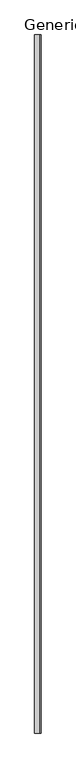
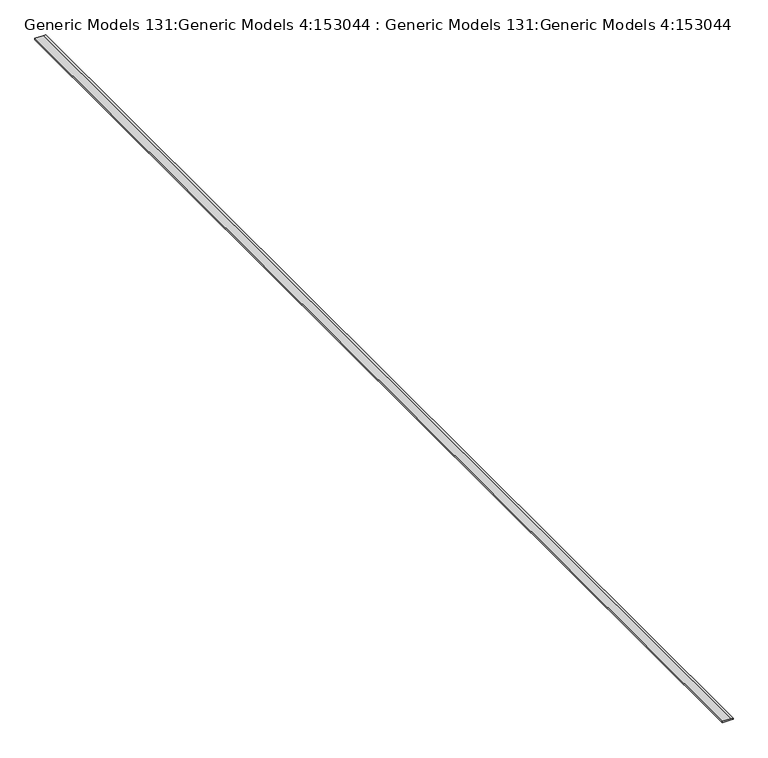
"""IFC4 building model written with IfcOpenShell, lengths in millimetres: proxy geometry, Generic Models 131:Generic Models 4:153044 : Generic Models 131:Generic Models 4:153044."""

from ifc_helpers import new_model, si_unit, frame, origin, place, context, project, spatial, polyline, outline, extrude, source, transform, mapped, element, save


def generic_models_131_generic_models_4_153044_generic_models_91a5e1c3(model_context):
    return source(origin(), model_context, "Body", "SweptSolid", [
        extrude(outline(polyline([(3067.05, 7068.698213), (3046.095, 7068.698213), (3046.095, 7091.141397), (3044.825, 7091.141397), (3044.825, 7231.429663), (3047.8274564, 7231.429663), (3047.8274564, 7232.699663), (3046.095, 7232.699663), (3046.095, 7234.909463), (3065.78, 7234.909463), (3065.78, 7198.079463), (3067.05, 7198.079463), (3067.05, 7068.698213)])), frame((0.0, -6674.7974793, 0.0), z_axis=(0.0, 1.0, 0.0), x_axis=(0.0, 0.0, 1.0)), (0.0, 0.0, 1.0), 18643.6),
    ])


if __name__ == "__main__":
    model = new_model("IFC4")
    model_context = context("Model", 3, world=origin())
    ifc_project = project(units=[si_unit("LENGTHUNIT", "METRE", prefix="MILLI")], contexts=[model_context])
    site = spatial("IfcSite", under=ifc_project)
    building = spatial("IfcBuilding", under=site)
    placement = place(None, origin())
    generic_models_131_generic_models_4_153044_generic_models_shape = generic_models_131_generic_models_4_153044_generic_models_91a5e1c3(model_context)
    element("IfcBuildingElementProxy", 1, Name="Generic Models 131:Generic Models 4:153044 : Generic Models 131:Generic Models 4:153044", ObjectType="Generic Models 131:Generic Models 4:153044 : Generic Models 131:Generic Models 4:153044", at=placement, inside=building, context=model_context, shape_type="MappedRepresentation", body=[
        mapped(generic_models_131_generic_models_4_153044_generic_models_shape, transform((0.0, 0.0, 0.0), x_axis=(1.0, 0.0, 0.0), y_axis=(0.0, 1.0, 0.0), z_axis=(0.0, 0.0, 1.0))),
    ])
    save(model, "model.ifc")

# Revit data of these elements
# Type "Generic Models 131:Generic Models 4:153044 : Generic Models 131:Generic Models 4:153044"
#   NameOverride = "Generic Models 131:Generic Models 4:153044"
#   ObjectTypeOverride = "Generic Models 131:Generic Models 4"
#   Reference = "Generic Models 4"
#   Category = "Generic Models"
#   Tag = "153044"
# Element 1 (IfcBuildingElementProxy, "Generic Models 131:Generic Models 4:153044 : Generic Models 131:Generic Models 4:153044")
#   Materials on its faces: "_7/8\" SMOOTH TROWEL EXTERIOR STUCCO (COLOR PER OWNER) 770"
# Materials
#   "_7/8\" SMOOTH TROWEL EXTERIOR STUCCO (COLOR PER OWNER) 770": class "Unassigned", colour RGB 233 233 233, transparency 0
